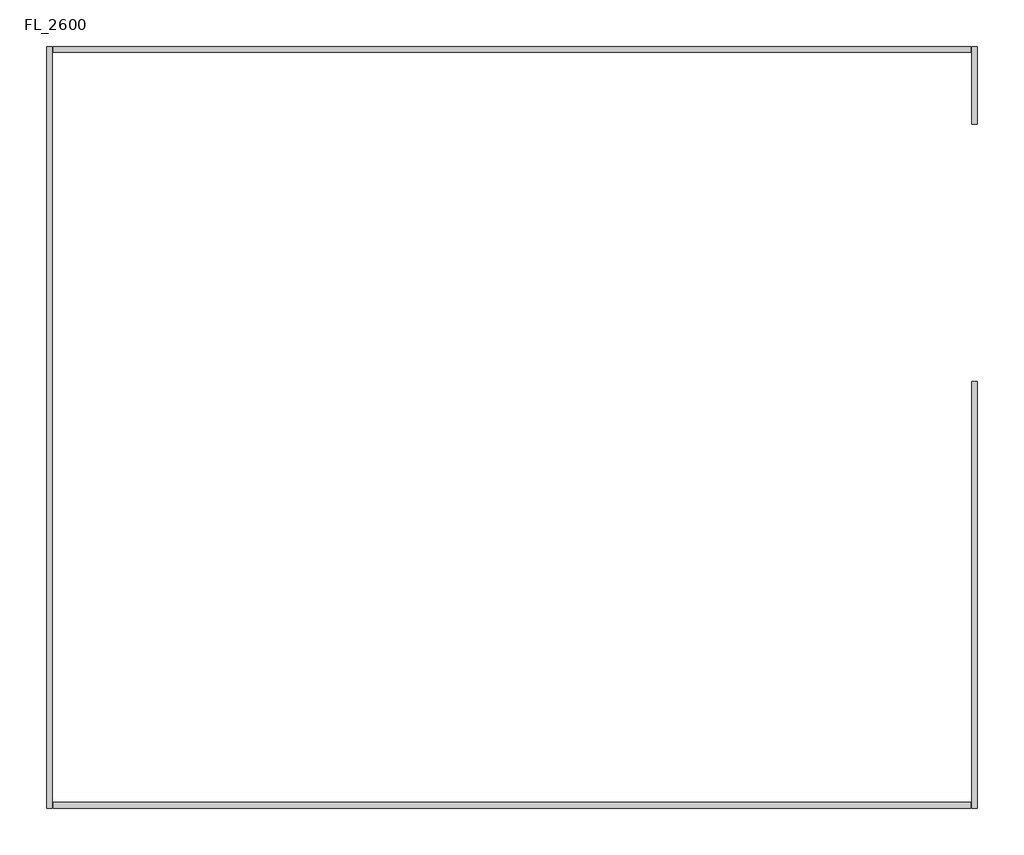
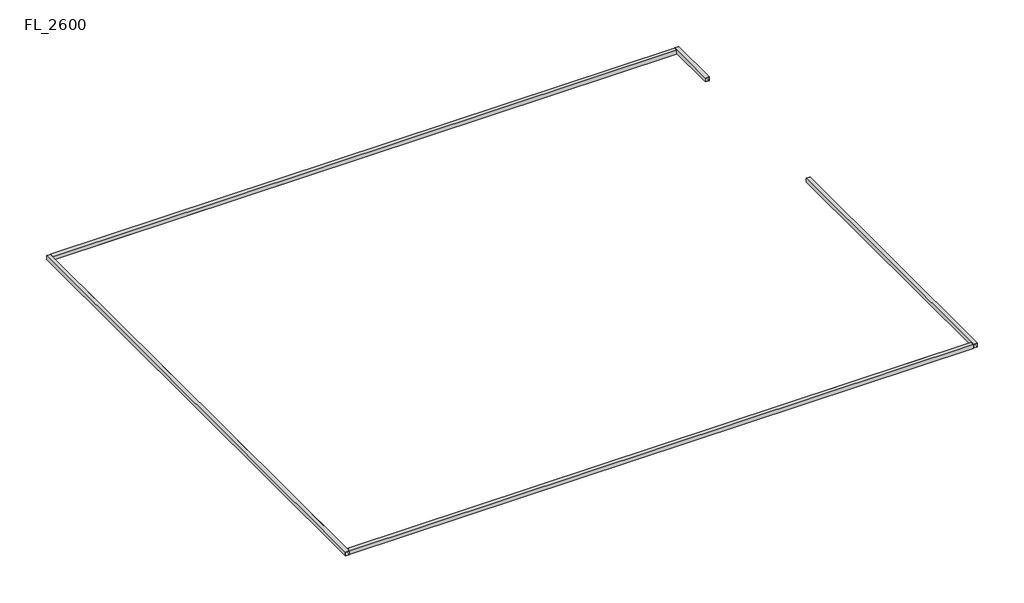
# One storey: 5 beams.
"""IFC4 building model written with IfcOpenShell, lengths in millimetres."""

import ifcopenshell
import ifcopenshell.guid

model = None  # the IFC model being written
_history = None  # IfcOwnerHistory: only IFC2X3 demands one
_inside = {}  # id of a spatial element -> (the spatial element, [elements in it])
_under = {}  # id of a project, library or spatial element -> (it, [spatial elements below it])
_declared = {}  # id of a project -> (the project, [libraries it declares])
_typed = {}  # id of a type object -> (the type object, [elements of that type])
_made_of = {}  # id of a material, layer set ... -> (it, [elements and type objects made of it])


def new_model(schema):
    """Start an empty IFC model of exactly this schema.

    Asked for "IFC4X3", IfcOpenShell would pick the latest addendum, in which some entities
    have other attributes; the version numbers below select the first issue.
    IFC2X3 requires an IfcOwnerHistory on every rooted entity: one is made here for all.
    """
    global model, _history
    if schema == "IFC4X3":
        model = ifcopenshell.file(schema_version=(4, 3, 0, 0))
    else:
        model = ifcopenshell.file(schema=schema)
    _inside.clear()
    _under.clear()
    _declared.clear()
    _typed.clear()
    _made_of.clear()
    _history = None
    if model.schema == "IFC2X3":
        org = make("IfcOrganization", Name="unknown")
        user = make(
            "IfcPersonAndOrganization",
            ThePerson=make("IfcPerson", FamilyName="unknown"),
            TheOrganization=org,
        )
        app = make(
            "IfcApplication",
            ApplicationDeveloper=org,
            Version="unknown",
            ApplicationFullName="unknown",
            ApplicationIdentifier="unknown",
        )
        _history = make(
            "IfcOwnerHistory",
            OwningUser=user,
            OwningApplication=app,
            ChangeAction="ADDED",
            CreationDate=0,
        )
    return model


def make(cls, **values):
    """One entity of the class cls with the attributes given. An attribute that is None is left unset."""
    return model.create_entity(
        cls, **{name: value for name, value in values.items() if value is not None}
    )


def rooted(cls, **values):
    """An entity with a GlobalId (a new one), such as an element, a storey or a relation."""
    return make(cls, GlobalId=ifcopenshell.guid.new(), OwnerHistory=_history, **values)


def si_unit(unit_type, name, prefix=None):
    """IfcSIUnit, for example si_unit("LENGTHUNIT", "METRE", prefix="MILLI")."""
    return make("IfcSIUnit", UnitType=unit_type, Prefix=prefix, Name=name)


def assignment(units):
    """IfcUnitAssignment: the units of a project."""
    return None if units is None else make("IfcUnitAssignment", Units=units)


def point(xyz):
    """IfcCartesianPoint."""
    return None if xyz is None else make("IfcCartesianPoint", Coordinates=xyz)


def direction(xyz):
    """IfcDirection."""
    return None if xyz is None else make("IfcDirection", DirectionRatios=xyz)


def frame(location, z_axis=None, x_axis=None):
    """IfcAxis2Placement3D, a coordinate frame: its origin and axes. An axis left out is left unset."""
    return make(
        "IfcAxis2Placement3D",
        Location=point(location),
        Axis=direction(z_axis),
        RefDirection=direction(x_axis),
    )


def origin():
    """The frame at (0, 0, 0) with its axes left unset."""
    return frame((0.0, 0.0, 0.0))


def place(relative_to, where):
    """IfcLocalPlacement: puts the frame where relative to a parent placement (None: the world)."""
    return make(
        "IfcLocalPlacement", PlacementRelTo=relative_to, RelativePlacement=where
    )


def context(
    kind, dimensions, precision=None, world=None, true_north=None, identifier=None
):
    """IfcGeometricRepresentationContext, for example the 3D "Model" context."""
    return make(
        "IfcGeometricRepresentationContext",
        ContextIdentifier=identifier,
        ContextType=kind,
        CoordinateSpaceDimension=dimensions,
        Precision=precision,
        WorldCoordinateSystem=world,
        TrueNorth=true_north,
    )


def project(units=None, contexts=None):
    """IfcProject with its units and contexts."""
    return rooted(
        "IfcProject",
        Name="project",
        RepresentationContexts=contexts,
        UnitsInContext=assignment(units),
    )


def spatial(cls, under=None, at=None, **own):
    """A site, building, storey or space (cls), placed at a placement, below another one or the project."""
    s = rooted(cls, ObjectPlacement=at, **own)
    if under is not None:
        _under.setdefault(under.id(), (under, []))[1].append(s)
    return s


def polyline(points):
    """IfcPolyline through the points."""
    return make("IfcPolyline", Points=[point(p) for p in points])


def outline(outer, holes=None, kind="AREA"):
    """IfcArbitraryClosedProfileDef: a profile drawn as a closed curve; with holes, ...WithVoids."""
    if holes is None:
        return make("IfcArbitraryClosedProfileDef", ProfileType=kind, OuterCurve=outer)
    return make(
        "IfcArbitraryProfileDefWithVoids",
        ProfileType=kind,
        OuterCurve=outer,
        InnerCurves=holes,
    )


def extrude(swept, where, along, depth):
    """IfcExtrudedAreaSolid: the profile swept, set in the frame where, extruded along a direction by depth."""
    return make(
        "IfcExtrudedAreaSolid",
        SweptArea=swept,
        Position=where,
        ExtrudedDirection=direction(along),
        Depth=depth,
    )


def shape(context_of_items, identifier, shape_type, items):
    """IfcShapeRepresentation: the items that make up one representation, for example the "Body"."""
    return make(
        "IfcShapeRepresentation",
        ContextOfItems=context_of_items,
        RepresentationIdentifier=identifier,
        RepresentationType=shape_type,
        Items=items,
    )


def source(mapping_origin, context_of_items, identifier, shape_type, items):
    """IfcRepresentationMap: a shape defined once, which mapped items show again and again."""
    return make(
        "IfcRepresentationMap",
        MappingOrigin=mapping_origin,
        MappedRepresentation=shape(context_of_items, identifier, shape_type, items),
    )


def transform(
    local_origin,
    x_axis=None,
    y_axis=None,
    z_axis=None,
    scale=None,
    scale2=None,
    scale3=None,
    uniform=True,
):
    """IfcCartesianTransformationOperator3D, or its non-uniform kind. x_axis, y_axis, z_axis: its Axis1, 2, 3."""
    if uniform:
        return make(
            "IfcCartesianTransformationOperator3D",
            Axis1=direction(x_axis),
            Axis2=direction(y_axis),
            LocalOrigin=point(local_origin),
            Scale=scale,
            Axis3=direction(z_axis),
        )
    return make(
        "IfcCartesianTransformationOperator3DnonUniform",
        Axis1=direction(x_axis),
        Axis2=direction(y_axis),
        LocalOrigin=point(local_origin),
        Scale=scale,
        Axis3=direction(z_axis),
        Scale2=scale2,
        Scale3=scale3,
    )


def mapped(mapping_source, mapping_target):
    """IfcMappedItem: shows the shape of a source again, moved by a transform."""
    return make(
        "IfcMappedItem", MappingSource=mapping_source, MappingTarget=mapping_target
    )


def made_of(thing, what):
    """Note that an element or type object is made of a material, layer set ...; save() writes the relation."""
    if what is not None:
        _made_of.setdefault(what.id(), (what, []))[1].append(thing)
    return thing


def element(
    cls,
    number,
    at=None,
    inside=None,
    cuts=None,
    type_object=None,
    material=None,
    context=None,
    identifier="Body",
    shape_type=None,
    held_by="IfcProductDefinitionShape",
    body=None,
    shapes=None,
    **own,
):
    """One element of the class cls, such as IfcWall. Its Tag is "e" and its number.

    at: its placement. inside: the storey or other place that contains it. cuts: it is an
    opening in that element (IfcRelVoidsElement). A single representation is given by context,
    identifier, shape_type and body (its items); several are given by shapes. held_by: the class
    of the entity that holds the representations. save() writes the other relations.
    """
    e = rooted(cls, Tag="e%d" % number, ObjectPlacement=at, **own)
    if body is not None:
        shapes = [shape(context, identifier, shape_type, body)]
    if shapes is not None:
        e.Representation = make(held_by, Representations=shapes)
    if inside is not None:
        _inside.setdefault(inside.id(), (inside, []))[1].append(e)
    if cuts is not None:
        rooted(
            "IfcRelVoidsElement", RelatingBuildingElement=cuts, RelatedOpeningElement=e
        )
    if type_object is not None:
        _typed.setdefault(type_object.id(), (type_object, []))[1].append(e)
    return made_of(e, material)


def aggregate(whole, parts):
    """IfcRelAggregates: a whole, such as a stair, and the parts it consists of."""
    return rooted("IfcRelAggregates", RelatingObject=whole, RelatedObjects=parts)


def save(model, path):
    """Write the relations noted so far, then the file.

    IfcRelAggregates (storeys below a building ...), IfcRelContainedInSpatialStructure (elements
    in a storey), IfcRelDefinesByType, IfcRelAssociatesMaterial and IfcRelDeclares: one each for
    every whole, place, type object, material and project.
    """
    for whole, parts in _under.values():
        aggregate(whole, parts)
    for where, things in _inside.values():
        rooted(
            "IfcRelContainedInSpatialStructure",
            RelatedElements=things,
            RelatingStructure=where,
        )
    for kind, things in _typed.values():
        rooted("IfcRelDefinesByType", RelatedObjects=things, RelatingType=kind)
    for what, things in _made_of.values():
        rooted("IfcRelAssociatesMaterial", RelatedObjects=things, RelatingMaterial=what)
    for by, libraries in _declared.values():
        rooted("IfcRelDeclares", RelatingContext=by, RelatedDefinitions=libraries)
    model.write(path)


def steel_rectangular_beam_bm125_rt_100x100x4_0_fd47acba(model_context):
    return source(origin(), model_context, "Body", "SweptSolid", [
        extrude(outline(polyline([(-50.0, 50.0), (50.0, 50.0), (50.0, -50.0), (-50.0, -50.0), (-50.0, 50.0)]), holes=[polyline([(46.0, -46.0), (46.0, 46.0), (-46.0, 46.0), (-46.0, -46.0), (46.0, -46.0)])]), frame((-7887.3, 0.0, 0.0), z_axis=(1.0, 0.0, 0.0), x_axis=(0.0, 1.0, 0.0)), (0.0, 0.0, 1.0), 15774.6),
        extrude(outline(polyline([(-50.0, 50.0), (50.0, 50.0), (50.0, -50.0), (-50.0, -50.0), (-50.0, 50.0)]), holes=[polyline([(46.0, -46.0), (46.0, 46.0), (-46.0, 46.0), (-46.0, -46.0), (46.0, -46.0)])]), frame((-7887.3, 0.0, 0.0), z_axis=(1.0, 0.0, 0.0), x_axis=(0.0, 1.0, 0.0)), (0.0, 0.0, 1.0), 15774.6),
        extrude(outline(polyline([(-50.0, 50.0), (50.0, 50.0), (50.0, -50.0), (-50.0, -50.0), (-50.0, 50.0)]), holes=[polyline([(46.0, -46.0), (46.0, 46.0), (-46.0, 46.0), (-46.0, -46.0), (46.0, -46.0)])]), frame((-7887.3, 0.0, 0.0), z_axis=(1.0, 0.0, 0.0), x_axis=(0.0, 1.0, 0.0)), (0.0, 0.0, 1.0), 15774.6),
        extrude(outline(polyline([(-50.0, 50.0), (50.0, 50.0), (50.0, -50.0), (-50.0, -50.0), (-50.0, 50.0)]), holes=[polyline([(46.0, -46.0), (46.0, 46.0), (-46.0, 46.0), (-46.0, -46.0), (46.0, -46.0)])]), frame((-7887.3, 0.0, 0.0), z_axis=(1.0, 0.0, 0.0), x_axis=(0.0, 1.0, 0.0)), (0.0, 0.0, 1.0), 15774.6),
    ])


def steel_rectangular_beam_bm125_rt_100x100x4_0_2c93a6f0(model_context):
    return source(origin(), model_context, "Body", "SweptSolid", [
        extrude(outline(polyline([(-50.0, 50.0), (50.0, 50.0), (50.0, -50.0), (-50.0, -50.0), (-50.0, 50.0)]), holes=[polyline([(46.0, -46.0), (46.0, 46.0), (-46.0, 46.0), (-46.0, -46.0), (46.0, -46.0)])]), frame((-6550.0, 0.0, 0.0), z_axis=(1.0, 0.0, 0.0), x_axis=(0.0, 1.0, 0.0)), (0.0, 0.0, 1.0), 13100.0),
        extrude(outline(polyline([(-50.0, 50.0), (50.0, 50.0), (50.0, -50.0), (-50.0, -50.0), (-50.0, 50.0)]), holes=[polyline([(46.0, -46.0), (46.0, 46.0), (-46.0, 46.0), (-46.0, -46.0), (46.0, -46.0)])]), frame((-6550.0, 0.0, 0.0), z_axis=(1.0, 0.0, 0.0), x_axis=(0.0, 1.0, 0.0)), (0.0, 0.0, 1.0), 13100.0),
        extrude(outline(polyline([(-50.0, 50.0), (50.0, 50.0), (50.0, -50.0), (-50.0, -50.0), (-50.0, 50.0)]), holes=[polyline([(46.0, -46.0), (46.0, 46.0), (-46.0, 46.0), (-46.0, -46.0), (46.0, -46.0)])]), frame((-6550.0, 0.0, 0.0), z_axis=(1.0, 0.0, 0.0), x_axis=(0.0, 1.0, 0.0)), (0.0, 0.0, 1.0), 13100.0),
        extrude(outline(polyline([(-50.0, 50.0), (50.0, 50.0), (50.0, -50.0), (-50.0, -50.0), (-50.0, 50.0)]), holes=[polyline([(46.0, -46.0), (46.0, 46.0), (-46.0, 46.0), (-46.0, -46.0), (46.0, -46.0)])]), frame((-6550.0, 0.0, 0.0), z_axis=(1.0, 0.0, 0.0), x_axis=(0.0, 1.0, 0.0)), (0.0, 0.0, 1.0), 13100.0),
    ])


def steel_rectangular_beam_bm125_rt_100x100x4_0_bbce7aa4(model_context):
    return source(origin(), model_context, "Body", "SweptSolid", [
        extrude(outline(polyline([(-50.0, 50.0), (50.0, 50.0), (50.0, -50.0), (-50.0, -50.0), (-50.0, 50.0)]), holes=[polyline([(46.0, -46.0), (46.0, 46.0), (-46.0, 46.0), (-46.0, -46.0), (46.0, -46.0)])]), frame((-3725.0, 0.0, 0.0), z_axis=(1.0, 0.0, 0.0), x_axis=(0.0, 1.0, 0.0)), (0.0, 0.0, 1.0), 7337.3),
        extrude(outline(polyline([(-50.0, 50.0), (50.0, 50.0), (50.0, -50.0), (-50.0, -50.0), (-50.0, 50.0)]), holes=[polyline([(46.0, -46.0), (46.0, 46.0), (-46.0, 46.0), (-46.0, -46.0), (46.0, -46.0)])]), frame((-3725.0, 0.0, 0.0), z_axis=(1.0, 0.0, 0.0), x_axis=(0.0, 1.0, 0.0)), (0.0, 0.0, 1.0), 7337.3),
        extrude(outline(polyline([(-50.0, 50.0), (50.0, 50.0), (50.0, -50.0), (-50.0, -50.0), (-50.0, 50.0)]), holes=[polyline([(46.0, -46.0), (46.0, 46.0), (-46.0, 46.0), (-46.0, -46.0), (46.0, -46.0)])]), frame((-3725.0, 0.0, 0.0), z_axis=(1.0, 0.0, 0.0), x_axis=(0.0, 1.0, 0.0)), (0.0, 0.0, 1.0), 7337.3),
        extrude(outline(polyline([(-50.0, 50.0), (50.0, 50.0), (50.0, -50.0), (-50.0, -50.0), (-50.0, 50.0)]), holes=[polyline([(46.0, -46.0), (46.0, 46.0), (-46.0, 46.0), (-46.0, -46.0), (46.0, -46.0)])]), frame((-3725.0, 0.0, 0.0), z_axis=(1.0, 0.0, 0.0), x_axis=(0.0, 1.0, 0.0)), (0.0, 0.0, 1.0), 7337.3),
    ])


def steel_rectangular_beam_bm125_rt_100x100x4_0_d4cde651(model_context):
    return source(origin(), model_context, "Body", "SweptSolid", [
        extrude(outline(polyline([(-50.0, 50.0), (50.0, 50.0), (50.0, -50.0), (-50.0, -50.0), (-50.0, 50.0)]), holes=[polyline([(46.0, -46.0), (46.0, 46.0), (-46.0, 46.0), (-46.0, -46.0), (46.0, -46.0)])]), frame((-612.3, 0.0, 0.0), z_axis=(1.0, 0.0, 0.0), x_axis=(0.0, 1.0, 0.0)), (0.0, 0.0, 1.0), 1337.3),
        extrude(outline(polyline([(-50.0, 50.0), (50.0, 50.0), (50.0, -50.0), (-50.0, -50.0), (-50.0, 50.0)]), holes=[polyline([(46.0, -46.0), (46.0, 46.0), (-46.0, 46.0), (-46.0, -46.0), (46.0, -46.0)])]), frame((-612.3, 0.0, 0.0), z_axis=(1.0, 0.0, 0.0), x_axis=(0.0, 1.0, 0.0)), (0.0, 0.0, 1.0), 1337.3),
        extrude(outline(polyline([(-50.0, 50.0), (50.0, 50.0), (50.0, -50.0), (-50.0, -50.0), (-50.0, 50.0)]), holes=[polyline([(46.0, -46.0), (46.0, 46.0), (-46.0, 46.0), (-46.0, -46.0), (46.0, -46.0)])]), frame((-612.3, 0.0, 0.0), z_axis=(1.0, 0.0, 0.0), x_axis=(0.0, 1.0, 0.0)), (0.0, 0.0, 1.0), 1337.3),
        extrude(outline(polyline([(-50.0, 50.0), (50.0, 50.0), (50.0, -50.0), (-50.0, -50.0), (-50.0, 50.0)]), holes=[polyline([(46.0, -46.0), (46.0, 46.0), (-46.0, 46.0), (-46.0, -46.0), (46.0, -46.0)])]), frame((-612.3, 0.0, 0.0), z_axis=(1.0, 0.0, 0.0), x_axis=(0.0, 1.0, 0.0)), (0.0, 0.0, 1.0), 1337.3),
    ])


model = new_model("IFC4")

# Units and contexts
model_context = context("Model", 3, world=origin())
ifc_project = project(units=[si_unit("LENGTHUNIT", "METRE", prefix="MILLI")], contexts=[model_context])

# Site, building, storey
site = spatial("IfcSite", under=ifc_project)
building = spatial("IfcBuilding", under=site)
storey = spatial("IfcBuildingStorey", under=building, Name="FL_2600", Elevation=2600.0)

# Beams
placement = place(None, origin())
steel_rectangular_beam_bm125_rt_100x100x4_0_shape = steel_rectangular_beam_bm125_rt_100x100x4_0_fd47acba(model_context)
element("IfcBeam", 1, ObjectType="Steel-Rectangular-Beam : BM125_RT-100x100x4.0", at=placement, inside=storey, context=model_context, shape_type="MappedRepresentation", body=[
    mapped(steel_rectangular_beam_bm125_rt_100x100x4_0_shape, transform((6100.0, 10094.5382614, 2550.0), x_axis=(1.0, 0.0, 0.0), y_axis=(0.0, 1.0, 0.0), z_axis=(0.0, 0.0, 1.0))),
])
element("IfcBeam", 2, ObjectType="Steel-Rectangular-Beam : BM125_RT-100x100x4.0", at=placement, inside=storey, context=model_context, shape_type="MappedRepresentation", body=[
    mapped(steel_rectangular_beam_bm125_rt_100x100x4_0_shape, transform((6100.0, 23094.5382614, 2550.0), x_axis=(-1.0, 0.0, 0.0), y_axis=(0.0, -1.0, 0.0), z_axis=(0.0, 0.0, 1.0))),
])
steel_rectangular_beam_bm125_rt_100x100x4_0_2_shape = steel_rectangular_beam_bm125_rt_100x100x4_0_2c93a6f0(model_context)
element("IfcBeam", 3, ObjectType="Steel-Rectangular-Beam : BM125_RT-100x100x4.0", at=placement, inside=storey, context=model_context, shape_type="MappedRepresentation", body=[
    mapped(steel_rectangular_beam_bm125_rt_100x100x4_0_2_shape, transform((-1850.0, 16594.5382614, 2550.0), x_axis=(0.0, -1.0, 0.0), y_axis=(1.0, 0.0, 0.0), z_axis=(0.0, 0.0, 1.0))),
])
steel_rectangular_beam_bm125_rt_100x100x4_0_3_shape = steel_rectangular_beam_bm125_rt_100x100x4_0_bbce7aa4(model_context)
element("IfcBeam", 4, ObjectType="Steel-Rectangular-Beam : BM125_RT-100x100x4.0", at=placement, inside=storey, context=model_context, shape_type="MappedRepresentation", body=[
    mapped(steel_rectangular_beam_bm125_rt_100x100x4_0_3_shape, transform((14050.0, 13769.5382614, 2550.0), x_axis=(0.0, 1.0, 0.0), y_axis=(-1.0, 0.0, 0.0), z_axis=(0.0, 0.0, 1.0))),
])
steel_rectangular_beam_bm125_rt_100x100x4_0_4_shape = steel_rectangular_beam_bm125_rt_100x100x4_0_d4cde651(model_context)
element("IfcBeam", 5, ObjectType="Steel-Rectangular-Beam : BM125_RT-100x100x4.0", at=placement, inside=storey, context=model_context, shape_type="MappedRepresentation", body=[
    mapped(steel_rectangular_beam_bm125_rt_100x100x4_0_4_shape, transform((14050.0, 22419.5382614, 2550.0), x_axis=(0.0, 1.0, 0.0), y_axis=(-1.0, 0.0, 0.0), z_axis=(0.0, 0.0, 1.0))),
])

save(model, "model.ifc")

# Revit data of these elements
# Type "Steel-Rectangular-Beam : BM125_RT-100x100x4.0"
#   t = 4 mm
#   Mass per Unit Length = 11.70 kg/m
#   Surface Area = 0.386 m²/m
#   Sectional Area = 14.95 cm²
#   Length [instance default] = 3000 mm
#   H = 100 mm
#   B = 100 mm
#   hec_material4 [instance default] = none
#   hec_material3 [instance default] = none
#   hec_material2 [instance default] = none
#   hec_material1 [instance default] = none
#   Structural Material [instance default] = none
# Elements 1, 2, 3, 4, 5 (IfcBeam, "Steel-Rectangular-Beam : BM125_RT-100x100x4.0")
#   Comments = ""
#   F01) Building Name = "Fire Water Pump Building"
#   F11) Project Building Tag_Type-1 = ""
#   F12) Project Building Tag_Type-2 = ""
#   F13) Project Facility Code = "621"
#   F21) Structural Type = "Steel"
#   F31) Standard Building Code = "E204"
#   F41) Discipline = "Architecture"
#   F51) Plan Start Date-Engineering = "2018-09-14"
#   F52) Plan Finish Date-Engineering = "2019-12-02"
#   F53) Duration = "444"
#   W11) Activity ID = "T3C621AR4110"
#   W12) Activity Name = "Fire Water Pump BLDG - Main Steel Structure"
#   W13) Plan Start Date = "2019-04-02"
#   W14) Plan Finish Date = "2019-06-03"
#   hec_material4 = none
#   hec_material3 = none
#   hec_material2 = S01AA010-00001_Main Steel Structure Fabrication Work_Shelter/Building_Steel Painting/Coating_for Non-Fireproofed Steel Surface, Surface Preparation, Primer, Second & Final Coat
#   hec_material1 = S03AA007-00001_Main Steel Structure Erection Work_Girth & Purlin
#   Structural Material = S01AA007-00001_Main Steel Structure Fabrication Work_Shelter/Building_Girth & Purlin
#   Phase Created = New Construction
#   Materials on its faces: "S01AA010-00001_Main Steel Structure Fabrication Work_Shelter/Building_Steel Painting/Coating_for Non-Fireproofed Steel Surface, Surface Preparation, Primer, Second & Final Coat"
# Materials
#   "S01AA010-00001_Main Steel Structure Fabrication Work_Shelter/Building_Steel Painting/Coating_for Non-Fireproofed Steel Surface, Surface Preparation, Primer, Second & Final Coat": class "Metal", colour RGB 120 120 120, transparency 0, Description = "Paint finished steel", W00) Work Master Code = "S01AA010-00001", W01) Work Master_Lv1 = "Main Steel Structure Fabrication Work", W02) Work Master_Lv2 = "Shelter/Building", W03) Work Master_Spec.1 = "Steel Painting/Coating", W04) Work Master_Spec.2 = "for Non-Fireproofed Steel Surface, Surface Preparation, Primer, Second & Final Coat", Cost = 0
#   "S03AA007-00001_Main Steel Structure Erection Work_Girth & Purlin": class "Metal", colour RGB 120 120 120, transparency 0, Comments = "(30KG/M>Weight)", Description = "Structural steel 50ksi", W00) Work Master Code = "S03AA007-00001", W01) Work Master_Lv1 = "Main Steel Structure Erection Work", W02) Work Master_Lv2 = "Shelter/Building", W03) Work Master_Spec.1 = "Girth & Purlin", Cost = 0
#   "S01AA007-00001_Main Steel Structure Fabrication Work_Shelter/Building_Girth & Purlin": class "Metal", colour RGB 120 120 120, transparency 0, Comments = "(30KG/M>Weight)", Description = "Structural steel 50ksi", W00) Work Master Code = "S01AA007-00001", W01) Work Master_Lv1 = "Main Steel Structure Fabrication Work", W02) Work Master_Lv2 = "Shelter/Building", W03) Work Master_Spec.1 = "Girth & Purlin", Cost = 0
